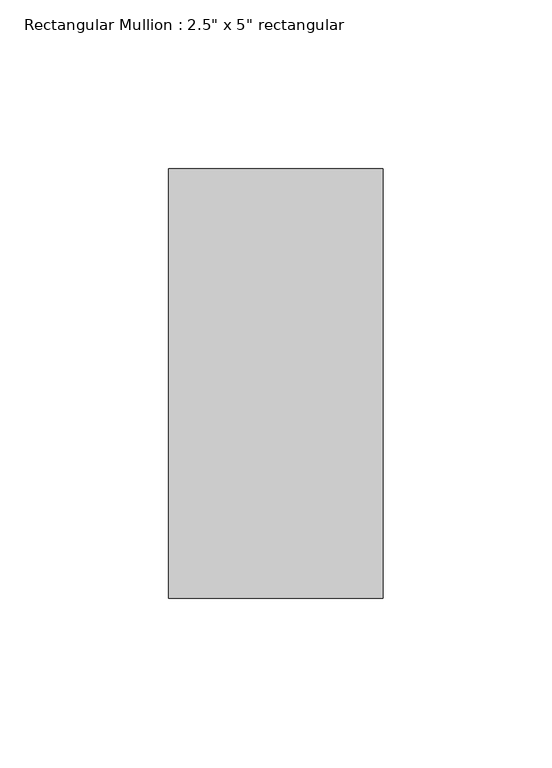
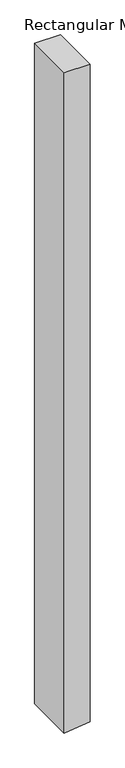
"""IFC4 building model written with IfcOpenShell, lengths in millimetres: member geometry."""

from ifc_helpers import new_model, si_unit, frame, origin, place, context, project, spatial, polyline, outline, extrude, source, transform, mapped, element, save


def member_9a6536ef(model_context):
    return source(origin(), model_context, "Body", "SweptSolid", [
        extrude(outline(polyline([(0.0, 31.75), (0.0, -31.75), (-1730.5709485, -31.75), (-1727.8092321, -7.0583463), (-1723.4685894, 31.75), (0.0, 31.75)])), frame((0.0, -63.5, 0.0), z_axis=(0.0, 1.0, 0.0), x_axis=(0.0, 0.0, 1.0)), (0.0, 0.0, 1.0), 127.0),
    ])


if __name__ == "__main__":
    model = new_model("IFC4")
    model_context = context("Model", 3, world=origin())
    ifc_project = project(units=[si_unit("LENGTHUNIT", "METRE", prefix="MILLI")], contexts=[model_context])
    site = spatial("IfcSite", under=ifc_project)
    building = spatial("IfcBuilding", under=site)
    placement = place(None, origin())
    member_shape = member_9a6536ef(model_context)
    element("IfcMember", 1, ObjectType="Rectangular Mullion : 2.5\" x 5\" rectangular", at=placement, inside=building, context=model_context, shape_type="MappedRepresentation", body=[
        mapped(member_shape, transform((0.0, 0.0, 0.0), x_axis=(1.0, 0.0, 0.0), y_axis=(0.0, 1.0, 0.0), z_axis=(0.0, 0.0, 1.0))),
    ])
    save(model, "model.ifc")

# Revit data of these elements
# Type "Rectangular Mullion : 2.5\" x 5\" rectangular"
#   built-in parameter 1007304 = 0.416667 (stored number, unit not read)
#   built-in parameter 1007301 = 0.104167 (stored number, unit not read)
#   built-in parameter 1007300 = 0.104167 (stored number, unit not read)
# Element 1 (IfcMember, "Rectangular Mullion : 2.5\" x 5\" rectangular")
#   Materials on its faces: "Aluminum"
# Materials
#   "Aluminum": class "Metal", colour RGB 247 247 247, transparency 0, Description = "Aluminum 6061", Cost = 0
